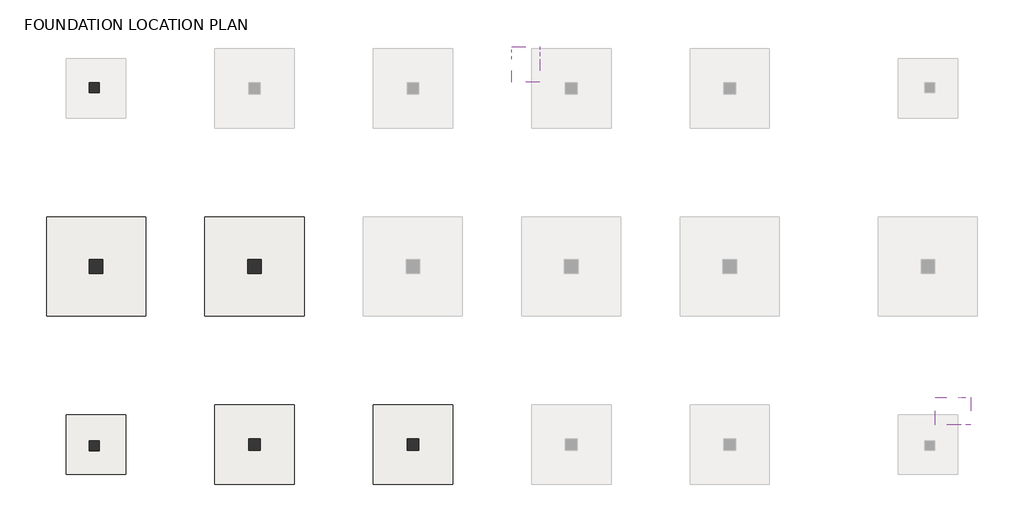
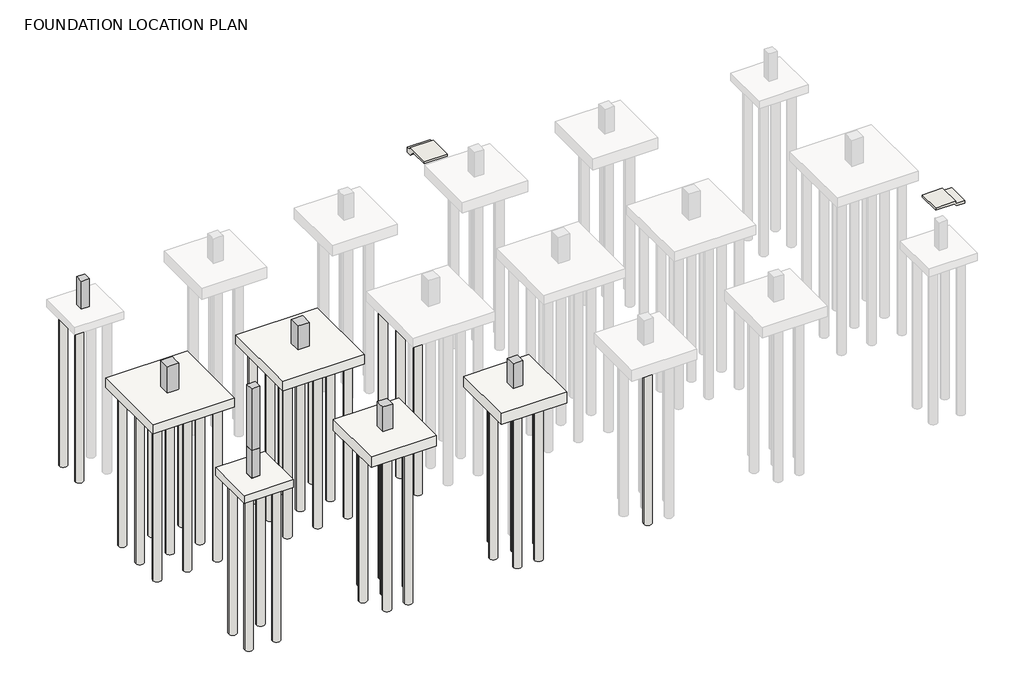
# One storey, part 1 of 3: 46 slabs, 7 columns, 2 walls.
"""IFC4 building model written with IfcOpenShell, lengths in millimetres."""

import ifcopenshell
import ifcopenshell.guid

model = None  # the IFC model being written
_history = None  # IfcOwnerHistory: only IFC2X3 demands one
_inside = {}  # id of a spatial element -> (the spatial element, [elements in it])
_under = {}  # id of a project, library or spatial element -> (it, [spatial elements below it])
_declared = {}  # id of a project -> (the project, [libraries it declares])
_typed = {}  # id of a type object -> (the type object, [elements of that type])
_made_of = {}  # id of a material, layer set ... -> (it, [elements and type objects made of it])


def new_model(schema):
    """Start an empty IFC model of exactly this schema.

    Asked for "IFC4X3", IfcOpenShell would pick the latest addendum, in which some entities
    have other attributes; the version numbers below select the first issue.
    IFC2X3 requires an IfcOwnerHistory on every rooted entity: one is made here for all.
    """
    global model, _history
    if schema == "IFC4X3":
        model = ifcopenshell.file(schema_version=(4, 3, 0, 0))
    else:
        model = ifcopenshell.file(schema=schema)
    _inside.clear()
    _under.clear()
    _declared.clear()
    _typed.clear()
    _made_of.clear()
    _history = None
    if model.schema == "IFC2X3":
        org = make("IfcOrganization", Name="unknown")
        user = make(
            "IfcPersonAndOrganization",
            ThePerson=make("IfcPerson", FamilyName="unknown"),
            TheOrganization=org,
        )
        app = make(
            "IfcApplication",
            ApplicationDeveloper=org,
            Version="unknown",
            ApplicationFullName="unknown",
            ApplicationIdentifier="unknown",
        )
        _history = make(
            "IfcOwnerHistory",
            OwningUser=user,
            OwningApplication=app,
            ChangeAction="ADDED",
            CreationDate=0,
        )
    return model


def make(cls, **values):
    """One entity of the class cls with the attributes given. An attribute that is None is left unset."""
    return model.create_entity(
        cls, **{name: value for name, value in values.items() if value is not None}
    )


def rooted(cls, **values):
    """An entity with a GlobalId (a new one), such as an element, a storey or a relation."""
    return make(cls, GlobalId=ifcopenshell.guid.new(), OwnerHistory=_history, **values)


def si_unit(unit_type, name, prefix=None):
    """IfcSIUnit, for example si_unit("LENGTHUNIT", "METRE", prefix="MILLI")."""
    return make("IfcSIUnit", UnitType=unit_type, Prefix=prefix, Name=name)


def assignment(units):
    """IfcUnitAssignment: the units of a project."""
    return None if units is None else make("IfcUnitAssignment", Units=units)


def point(xyz):
    """IfcCartesianPoint."""
    return None if xyz is None else make("IfcCartesianPoint", Coordinates=xyz)


def direction(xyz):
    """IfcDirection."""
    return None if xyz is None else make("IfcDirection", DirectionRatios=xyz)


def frame(location, z_axis=None, x_axis=None):
    """IfcAxis2Placement3D, a coordinate frame: its origin and axes. An axis left out is left unset."""
    return make(
        "IfcAxis2Placement3D",
        Location=point(location),
        Axis=direction(z_axis),
        RefDirection=direction(x_axis),
    )


def frame_2d(location, x_axis=None):
    """IfcAxis2Placement2D, a coordinate frame in the plane: its origin and x axis."""
    return make(
        "IfcAxis2Placement2D", Location=point(location), RefDirection=direction(x_axis)
    )


def origin():
    """The frame at (0, 0, 0) with its axes left unset."""
    return frame((0.0, 0.0, 0.0))


def place(relative_to, where):
    """IfcLocalPlacement: puts the frame where relative to a parent placement (None: the world)."""
    return make(
        "IfcLocalPlacement", PlacementRelTo=relative_to, RelativePlacement=where
    )


def context(
    kind, dimensions, precision=None, world=None, true_north=None, identifier=None
):
    """IfcGeometricRepresentationContext, for example the 3D "Model" context."""
    return make(
        "IfcGeometricRepresentationContext",
        ContextIdentifier=identifier,
        ContextType=kind,
        CoordinateSpaceDimension=dimensions,
        Precision=precision,
        WorldCoordinateSystem=world,
        TrueNorth=true_north,
    )


def project(units=None, contexts=None):
    """IfcProject with its units and contexts."""
    return rooted(
        "IfcProject",
        Name="project",
        RepresentationContexts=contexts,
        UnitsInContext=assignment(units),
    )


def spatial(cls, under=None, at=None, **own):
    """A site, building, storey or space (cls), placed at a placement, below another one or the project."""
    s = rooted(cls, ObjectPlacement=at, **own)
    if under is not None:
        _under.setdefault(under.id(), (under, []))[1].append(s)
    return s


def polyline(points):
    """IfcPolyline through the points."""
    return make("IfcPolyline", Points=[point(p) for p in points])


def circle_curve(where, radius):
    """IfcCircle in the frame where."""
    return make("IfcCircle", Position=where, Radius=radius)


def trimmed(basis, trim1, trim2, sense, master):
    """IfcTrimmedCurve: the piece of a basis curve between two trims."""
    return make(
        "IfcTrimmedCurve",
        BasisCurve=basis,
        Trim1=trim1,
        Trim2=trim2,
        SenseAgreement=sense,
        MasterRepresentation=master,
    )


def segment(curve, same_sense, transition):
    """IfcCompositeCurveSegment."""
    return make(
        "IfcCompositeCurveSegment",
        Transition=transition,
        SameSense=same_sense,
        ParentCurve=curve,
    )


def composite_curve(segments, self_intersect=None):
    """IfcCompositeCurve: segments joined end to end."""
    return make("IfcCompositeCurve", Segments=segments, SelfIntersect=self_intersect)


def outline(outer, holes=None, kind="AREA"):
    """IfcArbitraryClosedProfileDef: a profile drawn as a closed curve; with holes, ...WithVoids."""
    if holes is None:
        return make("IfcArbitraryClosedProfileDef", ProfileType=kind, OuterCurve=outer)
    return make(
        "IfcArbitraryProfileDefWithVoids",
        ProfileType=kind,
        OuterCurve=outer,
        InnerCurves=holes,
    )


def extrude(swept, where, along, depth):
    """IfcExtrudedAreaSolid: the profile swept, set in the frame where, extruded along a direction by depth."""
    return make(
        "IfcExtrudedAreaSolid",
        SweptArea=swept,
        Position=where,
        ExtrudedDirection=direction(along),
        Depth=depth,
    )


def faces_of(points, faces, orient=None, outer=None):
    """IfcFace entities. A face is a list of loops; a loop is a list of indices into points, from 0.

    orient and outer hold one flag for each loop. By default every Orientation is true, the
    first loop of a face is its IfcFaceOuterBound and the others are IfcFaceBound.
    """
    made = []
    for i, loops in enumerate(faces):
        bounds = []
        for j, loop in enumerate(loops):
            is_outer = j == 0 if outer is None else outer[i][j]
            bounds.append(
                make(
                    "IfcFaceOuterBound" if is_outer else "IfcFaceBound",
                    Bound=make("IfcPolyLoop", Polygon=[points[k] for k in loop]),
                    Orientation=True if orient is None else orient[i][j],
                )
            )
        made.append(make("IfcFace", Bounds=bounds))
    return made


def faceted_brep(points, faces, orient=None, outer=None, voids=None):
    """IfcFacetedBrep: a solid bounded by flat faces; with voids (closed shells), ...WithVoids."""
    shared = [point(p) for p in points]
    hull = make("IfcClosedShell", CfsFaces=faces_of(shared, faces, orient, outer))
    if voids is None:
        return make("IfcFacetedBrep", Outer=hull)
    return make(
        "IfcFacetedBrepWithVoids",
        Outer=hull,
        Voids=[
            make(cls, CfsFaces=faces_of(shared, fs, o, b)) for cls, fs, o, b in voids
        ],
    )


def shape(context_of_items, identifier, shape_type, items):
    """IfcShapeRepresentation: the items that make up one representation, for example the "Body"."""
    return make(
        "IfcShapeRepresentation",
        ContextOfItems=context_of_items,
        RepresentationIdentifier=identifier,
        RepresentationType=shape_type,
        Items=items,
    )


def source(mapping_origin, context_of_items, identifier, shape_type, items):
    """IfcRepresentationMap: a shape defined once, which mapped items show again and again."""
    return make(
        "IfcRepresentationMap",
        MappingOrigin=mapping_origin,
        MappedRepresentation=shape(context_of_items, identifier, shape_type, items),
    )


def transform(
    local_origin,
    x_axis=None,
    y_axis=None,
    z_axis=None,
    scale=None,
    scale2=None,
    scale3=None,
    uniform=True,
):
    """IfcCartesianTransformationOperator3D, or its non-uniform kind. x_axis, y_axis, z_axis: its Axis1, 2, 3."""
    if uniform:
        return make(
            "IfcCartesianTransformationOperator3D",
            Axis1=direction(x_axis),
            Axis2=direction(y_axis),
            LocalOrigin=point(local_origin),
            Scale=scale,
            Axis3=direction(z_axis),
        )
    return make(
        "IfcCartesianTransformationOperator3DnonUniform",
        Axis1=direction(x_axis),
        Axis2=direction(y_axis),
        LocalOrigin=point(local_origin),
        Scale=scale,
        Axis3=direction(z_axis),
        Scale2=scale2,
        Scale3=scale3,
    )


def mapped(mapping_source, mapping_target):
    """IfcMappedItem: shows the shape of a source again, moved by a transform."""
    return make(
        "IfcMappedItem", MappingSource=mapping_source, MappingTarget=mapping_target
    )


def made_of(thing, what):
    """Note that an element or type object is made of a material, layer set ...; save() writes the relation."""
    if what is not None:
        _made_of.setdefault(what.id(), (what, []))[1].append(thing)
    return thing


def element(
    cls,
    number,
    at=None,
    inside=None,
    cuts=None,
    type_object=None,
    material=None,
    context=None,
    identifier="Body",
    shape_type=None,
    held_by="IfcProductDefinitionShape",
    body=None,
    shapes=None,
    **own,
):
    """One element of the class cls, such as IfcWall. Its Tag is "e" and its number.

    at: its placement. inside: the storey or other place that contains it. cuts: it is an
    opening in that element (IfcRelVoidsElement). A single representation is given by context,
    identifier, shape_type and body (its items); several are given by shapes. held_by: the class
    of the entity that holds the representations. save() writes the other relations.
    """
    e = rooted(cls, Tag="e%d" % number, ObjectPlacement=at, **own)
    if body is not None:
        shapes = [shape(context, identifier, shape_type, body)]
    if shapes is not None:
        e.Representation = make(held_by, Representations=shapes)
    if inside is not None:
        _inside.setdefault(inside.id(), (inside, []))[1].append(e)
    if cuts is not None:
        rooted(
            "IfcRelVoidsElement", RelatingBuildingElement=cuts, RelatedOpeningElement=e
        )
    if type_object is not None:
        _typed.setdefault(type_object.id(), (type_object, []))[1].append(e)
    return made_of(e, material)


def aggregate(whole, parts):
    """IfcRelAggregates: a whole, such as a stair, and the parts it consists of."""
    return rooted("IfcRelAggregates", RelatingObject=whole, RelatedObjects=parts)


def save(model, path):
    """Write the relations noted so far, then the file.

    IfcRelAggregates (storeys below a building ...), IfcRelContainedInSpatialStructure (elements
    in a storey), IfcRelDefinesByType, IfcRelAssociatesMaterial and IfcRelDeclares: one each for
    every whole, place, type object, material and project.
    """
    for whole, parts in _under.values():
        aggregate(whole, parts)
    for where, things in _inside.values():
        rooted(
            "IfcRelContainedInSpatialStructure",
            RelatedElements=things,
            RelatingStructure=where,
        )
    for kind, things in _typed.values():
        rooted("IfcRelDefinesByType", RelatedObjects=things, RelatingType=kind)
    for what, things in _made_of.values():
        rooted("IfcRelAssociatesMaterial", RelatedObjects=things, RelatingMaterial=what)
    for by, libraries in _declared.values():
        rooted("IfcRelDeclares", RelatingContext=by, RelatedDefinitions=libraries)
    model.write(path)


def wall_a06d278e(model_context):
    return source(origin(), model_context, "Body", "SweptSolid", [
        extrude(outline(polyline([(599.905241, 43602.1335861), (599.905241, 42370.0), (449.905241, 42370.0), (449.905241, 43520.0), (299.905241, 43670.0), (299.905241, 44170.4893475), (449.905241, 44170.4893475), (449.905241, 43602.1335861), (599.905241, 43602.1335861)])), frame((0.0, 21999.5208589, 0.0), z_axis=(0.0, 1.0, 0.0), x_axis=(0.0, 0.0, 1.0)), (0.0, 0.0, 1.0), 1400.0),
    ])


def wall_c40cd3bd(model_context):
    return source(origin(), model_context, "Body", "SweptSolid", [
        extrude(outline(polyline([(40819.5208589, 599.905241), (40819.5208589, 449.905241), (41119.5208589, 449.905241), (41119.5208589, 109.2314637), (40810.1946362, 109.2314637), (40469.5208589, 449.905241), (39319.5208589, 449.905241), (39319.5208589, 599.905241), (40819.5208589, 599.905241)])), frame((21000.0, 0.0, 0.0), z_axis=(1.0, 0.0, 0.0), x_axis=(0.0, 1.0, 0.0)), (0.0, 0.0, 1.0), 1400.0),
    ])


model = new_model("IFC4")

# Units and contexts
model_context = context("Model", 3, world=origin())
ifc_project = project(units=[si_unit("LENGTHUNIT", "METRE", prefix="MILLI")], contexts=[model_context])

# Site, building, storey
site = spatial("IfcSite", under=ifc_project)
building = spatial("IfcBuilding", under=site)
storey = spatial("IfcBuildingStorey", under=building, Name="FOUNDATION LOCATION PLAN", Elevation=-1699.994759)

# Columns
placement = place(None, origin())
element("IfcColumn", 1, ObjectType="Concrete-Rectangular-Column_R1 : CLS113_RC COLUMN_AG_C1", at=placement, inside=storey, context=model_context, shape_type="Brep", body=[
    faceted_brep([(-350.0, 21199.5208589, -1699.994759), (150.0, 21199.5208589, -1699.994759), (150.0, 20699.5208589, -1699.994759), (-350.0, 20699.5208589, -1699.994759), (150.0, 21199.5208589, -1199.994759), (-350.0, 21199.5208589, -1199.994759), (-350.0, 20699.5208589, -1199.994759), (150.0, 20699.5208589, -1199.994759)], [[[0, 1, 2, 3]], [[4, 5, 6, 7]], [[1, 0, 5, 4]], [[2, 1, 4, 7]], [[3, 2, 7, 6]], [[0, 3, 6, 5]]]),
    faceted_brep([(-350.0, 21199.5208589, 4600.005241), (150.0, 21199.5208589, 4600.005241), (150.0, 21199.5208589, 600.005241), (-99.0, 21199.5208589, 600.005241), (-350.0, 21199.5208589, 600.005241), (-350.0, 21199.5208589, 3950.005241), (-350.0, 21199.5208589, 4550.005241), (150.0, 20699.5208589, 4600.005241), (150.0, 20699.5208589, 4550.005241), (150.0, 20699.5208589, 3950.005241), (150.0, 20699.5208589, 600.005241), (150.0, 20950.5208589, 600.005241), (-350.0, 20699.5208589, 4600.005241), (-350.0, 20699.5208589, 4550.005241), (-350.0, 20699.5208589, 3950.005241), (-350.0, 20699.5208589, 600.005241)], [[[0, 1, 2, 3, 4, 5, 6]], [[1, 7, 8, 9, 10, 11, 2]], [[7, 12, 13, 14, 15, 10, 9, 8]], [[12, 0, 6, 5, 4, 15, 14, 13]], [[1, 0, 12, 7]], [[4, 3, 2, 11, 10, 15]]]),
])
element("IfcColumn", 2, ObjectType="Concrete-Rectangular-Column_R1 : CLS111_RC COLUMN_UG_C1", at=placement, inside=storey, context=model_context, shape_type="Brep", body=[
    faceted_brep([(-350.0, 21199.5208589, -1199.994759), (150.0, 21199.5208589, -1199.994759), (150.0, 20699.5208589, -1199.994759), (-350.0, 20699.5208589, -1199.994759), (-350.0, 21199.5208589, 450.005241), (-350.0, 21199.5208589, 600.005241), (150.0, 21199.5208589, 600.005241), (150.0, 21199.5208589, 450.005241), (150.0, 20699.5208589, 600.005241), (150.0, 20699.5208589, 450.005241), (-350.0, 20699.5208589, 600.005241)], [[[0, 1, 2, 3]], [[1, 0, 4, 5, 6, 7]], [[2, 1, 7, 6, 8, 9]], [[3, 2, 9, 8, 10]], [[0, 3, 10, 5, 4]], [[6, 5, 10, 8]]]),
])
element("IfcColumn", 3, ObjectType="Concrete-Rectangular-Column_R1 : CLS111_RC COLUMN_UG_C1", at=placement, inside=storey, context=model_context, shape_type="Brep", body=[
    faceted_brep([(-350.0, 39299.5208589, -1199.994759), (150.0, 39299.5208589, -1199.994759), (150.0, 38799.5208589, -1199.994759), (-350.0, 38799.5208589, -1199.994759), (-350.0, 39299.5208589, 600.005241), (150.0, 39299.5208589, 600.005241), (150.0, 38999.7368538, 600.005241), (150.0, 38799.7368538, 600.005241), (150.0, 38799.5208589, 600.005241), (150.0, 38799.5208589, 450.005241), (0.0, 38799.5208589, 600.005241), (-350.0, 38799.5208589, 600.005241), (-350.0, 38799.7368538, 600.005241)], [[[0, 1, 2, 3]], [[1, 0, 4, 5]], [[2, 1, 5, 6, 7, 8, 9]], [[3, 2, 9, 8, 10, 11]], [[0, 3, 11, 12, 4]], [[5, 4, 12, 11, 10, 8, 7, 6]]]),
])
element("IfcColumn", 4, ObjectType="Concrete-Rectangular-Column_R1 : CLS111_RC COLUMN_UG_C3", at=placement, inside=storey, context=model_context, shape_type="Brep", body=[
    faceted_brep([(-350.0, 30349.5208589, -1099.994759), (350.0, 30349.5208589, -1099.994759), (350.0, 29649.5208589, -1099.994759), (-350.0, 29649.5208589, -1099.994759), (-350.0, 30349.5208589, 600.005241), (0.0, 30349.5208589, 600.005241), (350.0, 30349.5208589, 600.005241), (350.0, 30349.5208589, 450.005241), (350.0, 29999.5208589, 600.005241), (350.0, 29649.5208589, 600.005241), (-99.0, 29649.5208589, 600.005241), (-350.0, 29649.5208589, 600.005241)], [[[0, 1, 2, 3]], [[1, 0, 4, 5, 6, 7]], [[2, 1, 7, 6, 8, 9]], [[3, 2, 9, 10, 11]], [[0, 3, 11, 4]], [[11, 10, 9, 8, 6, 5, 4]]]),
])
element("IfcColumn", 5, ObjectType="Concrete-Rectangular-Column_R1 : CLS111_RC COLUMN_UG_C3", at=placement, inside=storey, context=model_context, shape_type="SweptSolid", body=[
    extrude(outline(polyline([(7650.0, 30349.5208589), (8350.0, 30349.5208589), (8350.0, 29649.5208589), (7650.0, 29649.5208589), (7650.0, 30349.5208589)])), frame((0.0, 0.0, -1099.994759), z_axis=(0.0, 0.0, 1.0), x_axis=(1.0, 0.0, 0.0)), (0.0, 0.0, 1.0), 1550.0),
])
element("IfcColumn", 6, ObjectType="Concrete-Rectangular-Column_R1 : CLS111_RC COLUMN_UG_C2", at=placement, inside=storey, context=model_context, shape_type="Brep", body=[
    faceted_brep([(7700.0, 21299.5208589, -999.994759), (8300.0, 21299.5208589, -999.994759), (8300.0, 20699.5208589, -999.994759), (7700.0, 20699.5208589, -999.994759), (7700.0, 21299.5208589, 450.005241), (7700.0, 21299.5208589, 600.005241), (8300.0, 21299.5208589, 600.005241), (8300.0, 21299.5208589, 450.005241), (8300.0, 20999.5208589, 600.005241), (8300.0, 20699.5208589, 600.005241), (7700.0, 20699.5208589, 600.005241), (7700.0, 20999.5208589, 600.005241)], [[[0, 1, 2, 3]], [[1, 0, 4, 5, 6, 7]], [[2, 1, 7, 6, 8, 9]], [[3, 2, 9, 10]], [[0, 3, 10, 11, 5, 4]], [[6, 5, 11, 10, 9, 8]]]),
])
element("IfcColumn", 7, ObjectType="Concrete-Rectangular-Column_R1 : CLS111_RC COLUMN_UG_C2", at=placement, inside=storey, context=model_context, shape_type="Brep", body=[
    faceted_brep([(15700.0, 21299.5208589, -999.994759), (16300.0, 21299.5208589, -999.994759), (16300.0, 20699.5208589, -999.994759), (15700.0, 20699.5208589, -999.994759), (15700.0, 21299.5208589, 450.005241), (15700.0, 21299.5208589, 600.005241), (16300.0, 21299.5208589, 600.005241), (16300.0, 21299.5208589, 450.005241), (16300.0, 20999.5208589, 600.005241), (16300.0, 20699.5208589, 600.005241), (15700.0, 20699.5208589, 600.005241), (15700.0, 20999.5208589, 600.005241)], [[[0, 1, 2, 3]], [[1, 0, 4, 5, 6, 7]], [[2, 1, 7, 6, 8, 9]], [[3, 2, 9, 10]], [[0, 3, 10, 11, 5, 4]], [[6, 5, 11, 10, 9, 8]]]),
])

# Slabs
element("IfcSlab", 8, ObjectType="Footing-Rectangular_R1 : FTS301_Footing-Rectangular_3000x3000x500_F1", at=placement, inside=storey, context=model_context, shape_type="SweptSolid", body=[
    extrude(outline(polyline([(1500.0, 22499.5208589), (1500.0, 19499.5208589), (-1500.0, 19499.5208589), (-1500.0, 22499.5208589), (1500.0, 22499.5208589)])), frame((0.0, 0.0, -1699.994759), z_axis=(0.0, 0.0, 1.0), x_axis=(1.0, 0.0, 0.0)), (0.0, 0.0, 1.0), 500.0),
])
element("IfcSlab", 9, ObjectType="Footing-Rectangular_R1 : FTS301_Footing-Rectangular_4000x4000x700_F2", at=placement, inside=storey, context=model_context, shape_type="SweptSolid", body=[
    extrude(outline(polyline([(10000.0, 22999.5208589), (10000.0, 18999.5208589), (6000.0, 18999.5208589), (6000.0, 22999.5208589), (10000.0, 22999.5208589)])), frame((0.0, 0.0, -1699.994759), z_axis=(0.0, 0.0, 1.0), x_axis=(1.0, 0.0, 0.0)), (0.0, 0.0, 1.0), 700.0),
])
element("IfcSlab", 10, ObjectType="Footing-Rectangular_R1 : FTS301_Footing-Rectangular_4000x4000x700_F2", at=placement, inside=storey, context=model_context, shape_type="SweptSolid", body=[
    extrude(outline(polyline([(18000.0, 22999.5208589), (18000.0, 18999.5208589), (14000.0, 18999.5208589), (14000.0, 22999.5208589), (18000.0, 22999.5208589)])), frame((0.0, 0.0, -1699.994759), z_axis=(0.0, 0.0, 1.0), x_axis=(1.0, 0.0, 0.0)), (0.0, 0.0, 1.0), 700.0),
])
element("IfcSlab", 11, ObjectType="Footing-Rectangular_R1 : FTS301_Footing-Rectangular_5000x5000x600_F3", at=placement, inside=storey, context=model_context, shape_type="SweptSolid", body=[
    extrude(outline(polyline([(2500.0, 32499.5208589), (2500.0, 27499.5208589), (-2500.0, 27499.5208589), (-2500.0, 32499.5208589), (2500.0, 32499.5208589)])), frame((0.0, 0.0, -1699.994759), z_axis=(0.0, 0.0, 1.0), x_axis=(1.0, 0.0, 0.0)), (0.0, 0.0, 1.0), 600.0),
])
element("IfcSlab", 12, ObjectType="Footing-Rectangular_R1 : FTS301_Footing-Rectangular_5000x5000x600_F3", at=placement, inside=storey, context=model_context, shape_type="SweptSolid", body=[
    extrude(outline(polyline([(10500.0, 32499.5208589), (10500.0, 27499.5208589), (5500.0, 27499.5208589), (5500.0, 32499.5208589), (10500.0, 32499.5208589)])), frame((0.0, 0.0, -1699.994759), z_axis=(0.0, 0.0, 1.0), x_axis=(1.0, 0.0, 0.0)), (0.0, 0.0, 1.0), 600.0),
])
element("IfcSlab", 13, ObjectType="HEC_PILE : FTPS102_D500", at=placement, inside=storey, context=model_context, shape_type="SweptSolid", body=[
    extrude(outline(composite_curve([segment(trimmed(circle_curve(frame_2d((7350.0, 19649.5208589)), 250.0), [point((7600.0, 19649.5208589))], [point((7100.0, 19649.5208589))], False, "CARTESIAN"), True, "CONTINUOUS"), segment(trimmed(circle_curve(frame_2d((7350.0, 19649.5208589)), 250.0), [point((7100.0, 19649.5208589))], [point((7600.0, 19649.5208589))], False, "CARTESIAN"), True, "CONTINUOUS")], self_intersect=False)), frame((0.0, 0.0, -11749.994759), z_axis=(0.0, 0.0, 1.0), x_axis=(1.0, 0.0, 0.0)), (0.0, 0.0, 1.0), 10150.0),
])
element("IfcSlab", 14, ObjectType="HEC_PILE : FTPS102_D500", at=placement, inside=storey, context=model_context, shape_type="SweptSolid", body=[
    extrude(outline(composite_curve([segment(trimmed(circle_curve(frame_2d((8650.0, 19649.5208589)), 250.0), [point((8400.0, 19649.5208589))], [point((8900.0, 19649.5208589))], False, "CARTESIAN"), True, "CONTINUOUS"), segment(trimmed(circle_curve(frame_2d((8650.0, 19649.5208589)), 250.0), [point((8900.0, 19649.5208589))], [point((8400.0, 19649.5208589))], False, "CARTESIAN"), True, "CONTINUOUS")], self_intersect=False)), frame((0.0, 0.0, -11749.994759), z_axis=(0.0, 0.0, 1.0), x_axis=(1.0, 0.0, 0.0)), (0.0, 0.0, 1.0), 10150.0),
])
element("IfcSlab", 15, ObjectType="HEC_PILE : FTPS102_D500", at=placement, inside=storey, context=model_context, shape_type="SweptSolid", body=[
    extrude(outline(composite_curve([segment(trimmed(circle_curve(frame_2d((6650.0, 20999.5208589)), 250.0), [point((6900.0, 20999.5208589))], [point((6400.0, 20999.5208589))], False, "CARTESIAN"), True, "CONTINUOUS"), segment(trimmed(circle_curve(frame_2d((6650.0, 20999.5208589)), 250.0), [point((6400.0, 20999.5208589))], [point((6900.0, 20999.5208589))], False, "CARTESIAN"), True, "CONTINUOUS")], self_intersect=False)), frame((0.0, 0.0, -11749.994759), z_axis=(0.0, 0.0, 1.0), x_axis=(1.0, 0.0, 0.0)), (0.0, 0.0, 1.0), 10150.0),
])
element("IfcSlab", 16, ObjectType="HEC_PILE : FTPS102_D500", at=placement, inside=storey, context=model_context, shape_type="SweptSolid", body=[
    extrude(outline(composite_curve([segment(trimmed(circle_curve(frame_2d((8000.0, 20999.5208589)), 250.0), [point((8250.0, 20999.5208589))], [point((7750.0, 20999.5208589))], False, "CARTESIAN"), True, "CONTINUOUS"), segment(trimmed(circle_curve(frame_2d((8000.0, 20999.5208589)), 250.0), [point((7750.0, 20999.5208589))], [point((8250.0, 20999.5208589))], False, "CARTESIAN"), True, "CONTINUOUS")], self_intersect=False)), frame((0.0, 0.0, -11749.994759), z_axis=(0.0, 0.0, 1.0), x_axis=(1.0, 0.0, 0.0)), (0.0, 0.0, 1.0), 10150.0),
])
element("IfcSlab", 17, ObjectType="HEC_PILE : FTPS102_D500", at=placement, inside=storey, context=model_context, shape_type="SweptSolid", body=[
    extrude(outline(composite_curve([segment(trimmed(circle_curve(frame_2d((9350.0, 20999.5208589)), 250.0), [point((9100.0, 20999.5208589))], [point((9600.0, 20999.5208589))], False, "CARTESIAN"), True, "CONTINUOUS"), segment(trimmed(circle_curve(frame_2d((9350.0, 20999.5208589)), 250.0), [point((9600.0, 20999.5208589))], [point((9100.0, 20999.5208589))], False, "CARTESIAN"), True, "CONTINUOUS")], self_intersect=False)), frame((0.0, 0.0, -11749.994759), z_axis=(0.0, 0.0, 1.0), x_axis=(1.0, 0.0, 0.0)), (0.0, 0.0, 1.0), 10150.0),
])
element("IfcSlab", 18, ObjectType="HEC_PILE : FTPS102_D500", at=placement, inside=storey, context=model_context, shape_type="SweptSolid", body=[
    extrude(outline(composite_curve([segment(trimmed(circle_curve(frame_2d((7350.0, 22349.5208589)), 250.0), [point((7600.0, 22349.5208589))], [point((7100.0, 22349.5208589))], False, "CARTESIAN"), True, "CONTINUOUS"), segment(trimmed(circle_curve(frame_2d((7350.0, 22349.5208589)), 250.0), [point((7100.0, 22349.5208589))], [point((7600.0, 22349.5208589))], False, "CARTESIAN"), True, "CONTINUOUS")], self_intersect=False)), frame((0.0, 0.0, -11749.994759), z_axis=(0.0, 0.0, 1.0), x_axis=(1.0, 0.0, 0.0)), (0.0, 0.0, 1.0), 10150.0),
])
element("IfcSlab", 19, ObjectType="HEC_PILE : FTPS102_D500", at=placement, inside=storey, context=model_context, shape_type="SweptSolid", body=[
    extrude(outline(composite_curve([segment(trimmed(circle_curve(frame_2d((8650.0, 22349.5208589)), 250.0), [point((8400.0, 22349.5208589))], [point((8900.0, 22349.5208589))], False, "CARTESIAN"), True, "CONTINUOUS"), segment(trimmed(circle_curve(frame_2d((8650.0, 22349.5208589)), 250.0), [point((8900.0, 22349.5208589))], [point((8400.0, 22349.5208589))], False, "CARTESIAN"), True, "CONTINUOUS")], self_intersect=False)), frame((0.0, 0.0, -11749.994759), z_axis=(0.0, 0.0, 1.0), x_axis=(1.0, 0.0, 0.0)), (0.0, 0.0, 1.0), 10150.0),
])
element("IfcSlab", 20, ObjectType="HEC_PILE : FTPS102_D500", at=placement, inside=storey, context=model_context, shape_type="SweptSolid", body=[
    extrude(outline(composite_curve([segment(trimmed(circle_curve(frame_2d((-850.0, 39849.5208589)), 250.0), [point((-600.0, 39849.5208589))], [point((-1100.0, 39849.5208589))], False, "CARTESIAN"), True, "CONTINUOUS"), segment(trimmed(circle_curve(frame_2d((-850.0, 39849.5208589)), 250.0), [point((-1100.0, 39849.5208589))], [point((-600.0, 39849.5208589))], False, "CARTESIAN"), True, "CONTINUOUS")], self_intersect=False)), frame((0.0, 0.0, -11749.994759), z_axis=(0.0, 0.0, 1.0), x_axis=(1.0, 0.0, 0.0)), (0.0, 0.0, 1.0), 10150.0),
])
element("IfcSlab", 21, ObjectType="HEC_PILE : FTPS102_D500", at=placement, inside=storey, context=model_context, shape_type="SweptSolid", body=[
    extrude(outline(composite_curve([segment(trimmed(circle_curve(frame_2d((-850.0, 21849.5208589)), 250.0), [point((-600.0, 21849.5208589))], [point((-1100.0, 21849.5208589))], False, "CARTESIAN"), True, "CONTINUOUS"), segment(trimmed(circle_curve(frame_2d((-850.0, 21849.5208589)), 250.0), [point((-1100.0, 21849.5208589))], [point((-600.0, 21849.5208589))], False, "CARTESIAN"), True, "CONTINUOUS")], self_intersect=False)), frame((0.0, 0.0, -11749.994759), z_axis=(0.0, 0.0, 1.0), x_axis=(1.0, 0.0, 0.0)), (0.0, 0.0, 1.0), 10150.0),
])
element("IfcSlab", 22, ObjectType="HEC_PILE : FTPS102_D500", at=placement, inside=storey, context=model_context, shape_type="SweptSolid", body=[
    extrude(outline(composite_curve([segment(trimmed(circle_curve(frame_2d((850.0, 21849.5208589)), 250.0), [point((600.0, 21849.5208589))], [point((1100.0, 21849.5208589))], False, "CARTESIAN"), True, "CONTINUOUS"), segment(trimmed(circle_curve(frame_2d((850.0, 21849.5208589)), 250.0), [point((1100.0, 21849.5208589))], [point((600.0, 21849.5208589))], False, "CARTESIAN"), True, "CONTINUOUS")], self_intersect=False)), frame((0.0, 0.0, -11749.994759), z_axis=(0.0, 0.0, 1.0), x_axis=(1.0, 0.0, 0.0)), (0.0, 0.0, 1.0), 10150.0),
])
element("IfcSlab", 23, ObjectType="HEC_PILE : FTPS102_D500", at=placement, inside=storey, context=model_context, shape_type="SweptSolid", body=[
    extrude(outline(composite_curve([segment(trimmed(circle_curve(frame_2d((-850.0, 20149.5208589)), 250.0), [point((-600.0, 20149.5208589))], [point((-1100.0, 20149.5208589))], False, "CARTESIAN"), True, "CONTINUOUS"), segment(trimmed(circle_curve(frame_2d((-850.0, 20149.5208589)), 250.0), [point((-1100.0, 20149.5208589))], [point((-600.0, 20149.5208589))], False, "CARTESIAN"), True, "CONTINUOUS")], self_intersect=False)), frame((0.0, 0.0, -11749.994759), z_axis=(0.0, 0.0, 1.0), x_axis=(1.0, 0.0, 0.0)), (0.0, 0.0, 1.0), 10150.0),
])
element("IfcSlab", 24, ObjectType="HEC_PILE : FTPS102_D500", at=placement, inside=storey, context=model_context, shape_type="SweptSolid", body=[
    extrude(outline(composite_curve([segment(trimmed(circle_curve(frame_2d((850.0, 20149.5208589)), 250.0), [point((600.0, 20149.5208589))], [point((1100.0, 20149.5208589))], False, "CARTESIAN"), True, "CONTINUOUS"), segment(trimmed(circle_curve(frame_2d((850.0, 20149.5208589)), 250.0), [point((1100.0, 20149.5208589))], [point((600.0, 20149.5208589))], False, "CARTESIAN"), True, "CONTINUOUS")], self_intersect=False)), frame((0.0, 0.0, -11749.994759), z_axis=(0.0, 0.0, 1.0), x_axis=(1.0, 0.0, 0.0)), (0.0, 0.0, 1.0), 10150.0),
])
element("IfcSlab", 25, ObjectType="HEC_PILE : FTPS102_D500", at=placement, inside=storey, context=model_context, shape_type="SweptSolid", body=[
    extrude(outline(composite_curve([segment(trimmed(circle_curve(frame_2d((15350.0, 19649.5208589)), 250.0), [point((15600.0, 19649.5208589))], [point((15100.0, 19649.5208589))], False, "CARTESIAN"), True, "CONTINUOUS"), segment(trimmed(circle_curve(frame_2d((15350.0, 19649.5208589)), 250.0), [point((15100.0, 19649.5208589))], [point((15600.0, 19649.5208589))], False, "CARTESIAN"), True, "CONTINUOUS")], self_intersect=False)), frame((0.0, 0.0, -11749.994759), z_axis=(0.0, 0.0, 1.0), x_axis=(1.0, 0.0, 0.0)), (0.0, 0.0, 1.0), 10150.0),
])
element("IfcSlab", 26, ObjectType="HEC_PILE : FTPS102_D500", at=placement, inside=storey, context=model_context, shape_type="SweptSolid", body=[
    extrude(outline(composite_curve([segment(trimmed(circle_curve(frame_2d((16650.0, 19649.5208589)), 250.0), [point((16400.0, 19649.5208589))], [point((16900.0, 19649.5208589))], False, "CARTESIAN"), True, "CONTINUOUS"), segment(trimmed(circle_curve(frame_2d((16650.0, 19649.5208589)), 250.0), [point((16900.0, 19649.5208589))], [point((16400.0, 19649.5208589))], False, "CARTESIAN"), True, "CONTINUOUS")], self_intersect=False)), frame((0.0, 0.0, -11749.994759), z_axis=(0.0, 0.0, 1.0), x_axis=(1.0, 0.0, 0.0)), (0.0, 0.0, 1.0), 10150.0),
])
element("IfcSlab", 27, ObjectType="HEC_PILE : FTPS102_D500", at=placement, inside=storey, context=model_context, shape_type="SweptSolid", body=[
    extrude(outline(composite_curve([segment(trimmed(circle_curve(frame_2d((14650.0, 20999.5208589)), 250.0), [point((14900.0, 20999.5208589))], [point((14400.0, 20999.5208589))], False, "CARTESIAN"), True, "CONTINUOUS"), segment(trimmed(circle_curve(frame_2d((14650.0, 20999.5208589)), 250.0), [point((14400.0, 20999.5208589))], [point((14900.0, 20999.5208589))], False, "CARTESIAN"), True, "CONTINUOUS")], self_intersect=False)), frame((0.0, 0.0, -11749.994759), z_axis=(0.0, 0.0, 1.0), x_axis=(1.0, 0.0, 0.0)), (0.0, 0.0, 1.0), 10150.0),
])
element("IfcSlab", 28, ObjectType="HEC_PILE : FTPS102_D500", at=placement, inside=storey, context=model_context, shape_type="SweptSolid", body=[
    extrude(outline(composite_curve([segment(trimmed(circle_curve(frame_2d((16000.0, 20999.5208589)), 250.0), [point((16250.0, 20999.5208589))], [point((15750.0, 20999.5208589))], False, "CARTESIAN"), True, "CONTINUOUS"), segment(trimmed(circle_curve(frame_2d((16000.0, 20999.5208589)), 250.0), [point((15750.0, 20999.5208589))], [point((16250.0, 20999.5208589))], False, "CARTESIAN"), True, "CONTINUOUS")], self_intersect=False)), frame((0.0, 0.0, -11749.994759), z_axis=(0.0, 0.0, 1.0), x_axis=(1.0, 0.0, 0.0)), (0.0, 0.0, 1.0), 10150.0),
])
element("IfcSlab", 29, ObjectType="HEC_PILE : FTPS102_D500", at=placement, inside=storey, context=model_context, shape_type="SweptSolid", body=[
    extrude(outline(composite_curve([segment(trimmed(circle_curve(frame_2d((17350.0, 20999.5208589)), 250.0), [point((17100.0, 20999.5208589))], [point((17600.0, 20999.5208589))], False, "CARTESIAN"), True, "CONTINUOUS"), segment(trimmed(circle_curve(frame_2d((17350.0, 20999.5208589)), 250.0), [point((17600.0, 20999.5208589))], [point((17100.0, 20999.5208589))], False, "CARTESIAN"), True, "CONTINUOUS")], self_intersect=False)), frame((0.0, 0.0, -11749.994759), z_axis=(0.0, 0.0, 1.0), x_axis=(1.0, 0.0, 0.0)), (0.0, 0.0, 1.0), 10150.0),
])
element("IfcSlab", 30, ObjectType="HEC_PILE : FTPS102_D500", at=placement, inside=storey, context=model_context, shape_type="SweptSolid", body=[
    extrude(outline(composite_curve([segment(trimmed(circle_curve(frame_2d((15350.0, 22349.5208589)), 250.0), [point((15600.0, 22349.5208589))], [point((15100.0, 22349.5208589))], False, "CARTESIAN"), True, "CONTINUOUS"), segment(trimmed(circle_curve(frame_2d((15350.0, 22349.5208589)), 250.0), [point((15100.0, 22349.5208589))], [point((15600.0, 22349.5208589))], False, "CARTESIAN"), True, "CONTINUOUS")], self_intersect=False)), frame((0.0, 0.0, -11749.994759), z_axis=(0.0, 0.0, 1.0), x_axis=(1.0, 0.0, 0.0)), (0.0, 0.0, 1.0), 10150.0),
])
element("IfcSlab", 31, ObjectType="HEC_PILE : FTPS102_D500", at=placement, inside=storey, context=model_context, shape_type="SweptSolid", body=[
    extrude(outline(composite_curve([segment(trimmed(circle_curve(frame_2d((23350.0, 19649.5208589)), 250.0), [point((23600.0, 19649.5208589))], [point((23100.0, 19649.5208589))], False, "CARTESIAN"), True, "CONTINUOUS"), segment(trimmed(circle_curve(frame_2d((23350.0, 19649.5208589)), 250.0), [point((23100.0, 19649.5208589))], [point((23600.0, 19649.5208589))], False, "CARTESIAN"), True, "CONTINUOUS")], self_intersect=False)), frame((0.0, 0.0, -11749.994759), z_axis=(0.0, 0.0, 1.0), x_axis=(1.0, 0.0, 0.0)), (0.0, 0.0, 1.0), 10150.0),
])
element("IfcSlab", 32, ObjectType="HEC_PILE : FTPS102_D500", at=placement, inside=storey, context=model_context, shape_type="SweptSolid", body=[
    extrude(outline(composite_curve([segment(trimmed(circle_curve(frame_2d((-1850.0, 29999.5208589)), 250.0), [point((-1600.0, 29999.5208589))], [point((-2100.0, 29999.5208589))], False, "CARTESIAN"), True, "CONTINUOUS"), segment(trimmed(circle_curve(frame_2d((-1850.0, 29999.5208589)), 250.0), [point((-2100.0, 29999.5208589))], [point((-1600.0, 29999.5208589))], False, "CARTESIAN"), True, "CONTINUOUS")], self_intersect=False)), frame((0.0, 0.0, -11749.994759), z_axis=(0.0, 0.0, 1.0), x_axis=(1.0, 0.0, 0.0)), (0.0, 0.0, 1.0), 10150.0),
])
element("IfcSlab", 33, ObjectType="HEC_PILE : FTPS102_D500", at=placement, inside=storey, context=model_context, shape_type="SweptSolid", body=[
    extrude(outline(composite_curve([segment(trimmed(circle_curve(frame_2d((1850.0, 29999.5208589)), 250.0), [point((1600.0, 29999.5208589))], [point((2100.0, 29999.5208589))], False, "CARTESIAN"), True, "CONTINUOUS"), segment(trimmed(circle_curve(frame_2d((1850.0, 29999.5208589)), 250.0), [point((2100.0, 29999.5208589))], [point((1600.0, 29999.5208589))], False, "CARTESIAN"), True, "CONTINUOUS")], self_intersect=False)), frame((0.0, 0.0, -11749.994759), z_axis=(0.0, 0.0, 1.0), x_axis=(1.0, 0.0, 0.0)), (0.0, 0.0, 1.0), 10150.0),
])
element("IfcSlab", 34, ObjectType="HEC_PILE : FTPS102_D500", at=placement, inside=storey, context=model_context, shape_type="SweptSolid", body=[
    extrude(outline(composite_curve([segment(trimmed(circle_curve(frame_2d((0.0, 29999.5208589)), 250.0), [point((-250.0, 29999.5208589))], [point((250.0, 29999.5208589))], False, "CARTESIAN"), True, "CONTINUOUS"), segment(trimmed(circle_curve(frame_2d((0.0, 29999.5208589)), 250.0), [point((250.0, 29999.5208589))], [point((-250.0, 29999.5208589))], False, "CARTESIAN"), True, "CONTINUOUS")], self_intersect=False)), frame((0.0, 0.0, -11749.994759), z_axis=(0.0, 0.0, 1.0), x_axis=(1.0, 0.0, 0.0)), (0.0, 0.0, 1.0), 10150.0),
])
element("IfcSlab", 35, ObjectType="HEC_PILE : FTPS102_D500", at=placement, inside=storey, context=model_context, shape_type="SweptSolid", body=[
    extrude(outline(composite_curve([segment(trimmed(circle_curve(frame_2d((-1850.0, 31849.5208589)), 250.0), [point((-1600.0, 31849.5208589))], [point((-2100.0, 31849.5208589))], False, "CARTESIAN"), True, "CONTINUOUS"), segment(trimmed(circle_curve(frame_2d((-1850.0, 31849.5208589)), 250.0), [point((-2100.0, 31849.5208589))], [point((-1600.0, 31849.5208589))], False, "CARTESIAN"), True, "CONTINUOUS")], self_intersect=False)), frame((0.0, 0.0, -11749.994759), z_axis=(0.0, 0.0, 1.0), x_axis=(1.0, 0.0, 0.0)), (0.0, 0.0, 1.0), 10150.0),
])
element("IfcSlab", 36, ObjectType="HEC_PILE : FTPS102_D500", at=placement, inside=storey, context=model_context, shape_type="SweptSolid", body=[
    extrude(outline(composite_curve([segment(trimmed(circle_curve(frame_2d((1850.0, 31849.5208589)), 250.0), [point((1600.0, 31849.5208589))], [point((2100.0, 31849.5208589))], False, "CARTESIAN"), True, "CONTINUOUS"), segment(trimmed(circle_curve(frame_2d((1850.0, 31849.5208589)), 250.0), [point((2100.0, 31849.5208589))], [point((1600.0, 31849.5208589))], False, "CARTESIAN"), True, "CONTINUOUS")], self_intersect=False)), frame((0.0, 0.0, -11749.994759), z_axis=(0.0, 0.0, 1.0), x_axis=(1.0, 0.0, 0.0)), (0.0, 0.0, 1.0), 10150.0),
])
element("IfcSlab", 37, ObjectType="HEC_PILE : FTPS102_D500", at=placement, inside=storey, context=model_context, shape_type="SweptSolid", body=[
    extrude(outline(composite_curve([segment(trimmed(circle_curve(frame_2d((0.0, 31849.5208589)), 250.0), [point((-250.0, 31849.5208589))], [point((250.0, 31849.5208589))], False, "CARTESIAN"), True, "CONTINUOUS"), segment(trimmed(circle_curve(frame_2d((0.0, 31849.5208589)), 250.0), [point((250.0, 31849.5208589))], [point((-250.0, 31849.5208589))], False, "CARTESIAN"), True, "CONTINUOUS")], self_intersect=False)), frame((0.0, 0.0, -11749.994759), z_axis=(0.0, 0.0, 1.0), x_axis=(1.0, 0.0, 0.0)), (0.0, 0.0, 1.0), 10150.0),
])
element("IfcSlab", 38, ObjectType="HEC_PILE : FTPS102_D500", at=placement, inside=storey, context=model_context, shape_type="SweptSolid", body=[
    extrude(outline(composite_curve([segment(trimmed(circle_curve(frame_2d((-1850.0, 28149.5208589)), 250.0), [point((-1600.0, 28149.5208589))], [point((-2100.0, 28149.5208589))], False, "CARTESIAN"), True, "CONTINUOUS"), segment(trimmed(circle_curve(frame_2d((-1850.0, 28149.5208589)), 250.0), [point((-2100.0, 28149.5208589))], [point((-1600.0, 28149.5208589))], False, "CARTESIAN"), True, "CONTINUOUS")], self_intersect=False)), frame((0.0, 0.0, -11749.994759), z_axis=(0.0, 0.0, 1.0), x_axis=(1.0, 0.0, 0.0)), (0.0, 0.0, 1.0), 10150.0),
])
element("IfcSlab", 39, ObjectType="HEC_PILE : FTPS102_D500", at=placement, inside=storey, context=model_context, shape_type="SweptSolid", body=[
    extrude(outline(composite_curve([segment(trimmed(circle_curve(frame_2d((1850.0, 28149.5208589)), 250.0), [point((1600.0, 28149.5208589))], [point((2100.0, 28149.5208589))], False, "CARTESIAN"), True, "CONTINUOUS"), segment(trimmed(circle_curve(frame_2d((1850.0, 28149.5208589)), 250.0), [point((2100.0, 28149.5208589))], [point((1600.0, 28149.5208589))], False, "CARTESIAN"), True, "CONTINUOUS")], self_intersect=False)), frame((0.0, 0.0, -11749.994759), z_axis=(0.0, 0.0, 1.0), x_axis=(1.0, 0.0, 0.0)), (0.0, 0.0, 1.0), 10150.0),
])
element("IfcSlab", 40, ObjectType="HEC_PILE : FTPS102_D500", at=placement, inside=storey, context=model_context, shape_type="SweptSolid", body=[
    extrude(outline(composite_curve([segment(trimmed(circle_curve(frame_2d((0.0, 28149.5208589)), 250.0), [point((-250.0, 28149.5208589))], [point((250.0, 28149.5208589))], False, "CARTESIAN"), True, "CONTINUOUS"), segment(trimmed(circle_curve(frame_2d((0.0, 28149.5208589)), 250.0), [point((250.0, 28149.5208589))], [point((-250.0, 28149.5208589))], False, "CARTESIAN"), True, "CONTINUOUS")], self_intersect=False)), frame((0.0, 0.0, -11749.994759), z_axis=(0.0, 0.0, 1.0), x_axis=(1.0, 0.0, 0.0)), (0.0, 0.0, 1.0), 10150.0),
])
element("IfcSlab", 41, ObjectType="HEC_PILE : FTPS102_D500", at=placement, inside=storey, context=model_context, shape_type="SweptSolid", body=[
    extrude(outline(composite_curve([segment(trimmed(circle_curve(frame_2d((6150.0, 29999.5208589)), 250.0), [point((6400.0, 29999.5208589))], [point((5900.0, 29999.5208589))], False, "CARTESIAN"), True, "CONTINUOUS"), segment(trimmed(circle_curve(frame_2d((6150.0, 29999.5208589)), 250.0), [point((5900.0, 29999.5208589))], [point((6400.0, 29999.5208589))], False, "CARTESIAN"), True, "CONTINUOUS")], self_intersect=False)), frame((0.0, 0.0, -11749.994759), z_axis=(0.0, 0.0, 1.0), x_axis=(1.0, 0.0, 0.0)), (0.0, 0.0, 1.0), 10150.0),
])
element("IfcSlab", 42, ObjectType="HEC_PILE : FTPS102_D500", at=placement, inside=storey, context=model_context, shape_type="SweptSolid", body=[
    extrude(outline(composite_curve([segment(trimmed(circle_curve(frame_2d((9850.0, 29999.5208589)), 250.0), [point((9600.0, 29999.5208589))], [point((10100.0, 29999.5208589))], False, "CARTESIAN"), True, "CONTINUOUS"), segment(trimmed(circle_curve(frame_2d((9850.0, 29999.5208589)), 250.0), [point((10100.0, 29999.5208589))], [point((9600.0, 29999.5208589))], False, "CARTESIAN"), True, "CONTINUOUS")], self_intersect=False)), frame((0.0, 0.0, -11749.994759), z_axis=(0.0, 0.0, 1.0), x_axis=(1.0, 0.0, 0.0)), (0.0, 0.0, 1.0), 10150.0),
])
element("IfcSlab", 43, ObjectType="HEC_PILE : FTPS102_D500", at=placement, inside=storey, context=model_context, shape_type="SweptSolid", body=[
    extrude(outline(composite_curve([segment(trimmed(circle_curve(frame_2d((8000.0, 29999.5208589)), 250.0), [point((7750.0, 29999.5208589))], [point((8250.0, 29999.5208589))], False, "CARTESIAN"), True, "CONTINUOUS"), segment(trimmed(circle_curve(frame_2d((8000.0, 29999.5208589)), 250.0), [point((8250.0, 29999.5208589))], [point((7750.0, 29999.5208589))], False, "CARTESIAN"), True, "CONTINUOUS")], self_intersect=False)), frame((0.0, 0.0, -11749.994759), z_axis=(0.0, 0.0, 1.0), x_axis=(1.0, 0.0, 0.0)), (0.0, 0.0, 1.0), 10150.0),
])
element("IfcSlab", 44, ObjectType="HEC_PILE : FTPS102_D500", at=placement, inside=storey, context=model_context, shape_type="SweptSolid", body=[
    extrude(outline(composite_curve([segment(trimmed(circle_curve(frame_2d((6150.0, 31849.5208589)), 250.0), [point((6400.0, 31849.5208589))], [point((5900.0, 31849.5208589))], False, "CARTESIAN"), True, "CONTINUOUS"), segment(trimmed(circle_curve(frame_2d((6150.0, 31849.5208589)), 250.0), [point((5900.0, 31849.5208589))], [point((6400.0, 31849.5208589))], False, "CARTESIAN"), True, "CONTINUOUS")], self_intersect=False)), frame((0.0, 0.0, -11749.994759), z_axis=(0.0, 0.0, 1.0), x_axis=(1.0, 0.0, 0.0)), (0.0, 0.0, 1.0), 10150.0),
])
element("IfcSlab", 45, ObjectType="HEC_PILE : FTPS102_D500", at=placement, inside=storey, context=model_context, shape_type="SweptSolid", body=[
    extrude(outline(composite_curve([segment(trimmed(circle_curve(frame_2d((9850.0, 31849.5208589)), 250.0), [point((9600.0, 31849.5208589))], [point((10100.0, 31849.5208589))], False, "CARTESIAN"), True, "CONTINUOUS"), segment(trimmed(circle_curve(frame_2d((9850.0, 31849.5208589)), 250.0), [point((10100.0, 31849.5208589))], [point((9600.0, 31849.5208589))], False, "CARTESIAN"), True, "CONTINUOUS")], self_intersect=False)), frame((0.0, 0.0, -11749.994759), z_axis=(0.0, 0.0, 1.0), x_axis=(1.0, 0.0, 0.0)), (0.0, 0.0, 1.0), 10150.0),
])
element("IfcSlab", 46, ObjectType="HEC_PILE : FTPS102_D500", at=placement, inside=storey, context=model_context, shape_type="SweptSolid", body=[
    extrude(outline(composite_curve([segment(trimmed(circle_curve(frame_2d((8000.0, 31849.5208589)), 250.0), [point((7750.0, 31849.5208589))], [point((8250.0, 31849.5208589))], False, "CARTESIAN"), True, "CONTINUOUS"), segment(trimmed(circle_curve(frame_2d((8000.0, 31849.5208589)), 250.0), [point((8250.0, 31849.5208589))], [point((7750.0, 31849.5208589))], False, "CARTESIAN"), True, "CONTINUOUS")], self_intersect=False)), frame((0.0, 0.0, -11749.994759), z_axis=(0.0, 0.0, 1.0), x_axis=(1.0, 0.0, 0.0)), (0.0, 0.0, 1.0), 10150.0),
])
element("IfcSlab", 47, ObjectType="HEC_PILE : FTPS102_D500", at=placement, inside=storey, context=model_context, shape_type="SweptSolid", body=[
    extrude(outline(composite_curve([segment(trimmed(circle_curve(frame_2d((6150.0, 28149.5208589)), 250.0), [point((6400.0, 28149.5208589))], [point((5900.0, 28149.5208589))], False, "CARTESIAN"), True, "CONTINUOUS"), segment(trimmed(circle_curve(frame_2d((6150.0, 28149.5208589)), 250.0), [point((5900.0, 28149.5208589))], [point((6400.0, 28149.5208589))], False, "CARTESIAN"), True, "CONTINUOUS")], self_intersect=False)), frame((0.0, 0.0, -11749.994759), z_axis=(0.0, 0.0, 1.0), x_axis=(1.0, 0.0, 0.0)), (0.0, 0.0, 1.0), 10150.0),
])
element("IfcSlab", 48, ObjectType="HEC_PILE : FTPS102_D500", at=placement, inside=storey, context=model_context, shape_type="SweptSolid", body=[
    extrude(outline(composite_curve([segment(trimmed(circle_curve(frame_2d((9850.0, 28149.5208589)), 250.0), [point((9600.0, 28149.5208589))], [point((10100.0, 28149.5208589))], False, "CARTESIAN"), True, "CONTINUOUS"), segment(trimmed(circle_curve(frame_2d((9850.0, 28149.5208589)), 250.0), [point((10100.0, 28149.5208589))], [point((9600.0, 28149.5208589))], False, "CARTESIAN"), True, "CONTINUOUS")], self_intersect=False)), frame((0.0, 0.0, -11749.994759), z_axis=(0.0, 0.0, 1.0), x_axis=(1.0, 0.0, 0.0)), (0.0, 0.0, 1.0), 10150.0),
])
element("IfcSlab", 49, ObjectType="HEC_PILE : FTPS102_D500", at=placement, inside=storey, context=model_context, shape_type="SweptSolid", body=[
    extrude(outline(composite_curve([segment(trimmed(circle_curve(frame_2d((8000.0, 28149.5208589)), 250.0), [point((7750.0, 28149.5208589))], [point((8250.0, 28149.5208589))], False, "CARTESIAN"), True, "CONTINUOUS"), segment(trimmed(circle_curve(frame_2d((8000.0, 28149.5208589)), 250.0), [point((8250.0, 28149.5208589))], [point((7750.0, 28149.5208589))], False, "CARTESIAN"), True, "CONTINUOUS")], self_intersect=False)), frame((0.0, 0.0, -11749.994759), z_axis=(0.0, 0.0, 1.0), x_axis=(1.0, 0.0, 0.0)), (0.0, 0.0, 1.0), 10150.0),
])
element("IfcSlab", 50, ObjectType="HEC_PILE : FTPS102_D500", at=placement, inside=storey, context=model_context, shape_type="SweptSolid", body=[
    extrude(outline(composite_curve([segment(trimmed(circle_curve(frame_2d((14150.0, 29999.5208589)), 250.0), [point((14400.0, 29999.5208589))], [point((13900.0, 29999.5208589))], False, "CARTESIAN"), True, "CONTINUOUS"), segment(trimmed(circle_curve(frame_2d((14150.0, 29999.5208589)), 250.0), [point((13900.0, 29999.5208589))], [point((14400.0, 29999.5208589))], False, "CARTESIAN"), True, "CONTINUOUS")], self_intersect=False)), frame((0.0, 0.0, -11749.994759), z_axis=(0.0, 0.0, 1.0), x_axis=(1.0, 0.0, 0.0)), (0.0, 0.0, 1.0), 10150.0),
])
element("IfcSlab", 51, ObjectType="HEC_PILE : FTPS102_D500", at=placement, inside=storey, context=model_context, shape_type="SweptSolid", body=[
    extrude(outline(composite_curve([segment(trimmed(circle_curve(frame_2d((14150.0, 31849.5208589)), 250.0), [point((14400.0, 31849.5208589))], [point((13900.0, 31849.5208589))], False, "CARTESIAN"), True, "CONTINUOUS"), segment(trimmed(circle_curve(frame_2d((14150.0, 31849.5208589)), 250.0), [point((13900.0, 31849.5208589))], [point((14400.0, 31849.5208589))], False, "CARTESIAN"), True, "CONTINUOUS")], self_intersect=False)), frame((0.0, 0.0, -11749.994759), z_axis=(0.0, 0.0, 1.0), x_axis=(1.0, 0.0, 0.0)), (0.0, 0.0, 1.0), 10150.0),
])
element("IfcSlab", 52, ObjectType="HEC_PILE : FTPS102_D500", at=placement, inside=storey, context=model_context, shape_type="SweptSolid", body=[
    extrude(outline(composite_curve([segment(trimmed(circle_curve(frame_2d((14150.0, 28149.5208589)), 250.0), [point((14400.0, 28149.5208589))], [point((13900.0, 28149.5208589))], False, "CARTESIAN"), True, "CONTINUOUS"), segment(trimmed(circle_curve(frame_2d((14150.0, 28149.5208589)), 250.0), [point((13900.0, 28149.5208589))], [point((14400.0, 28149.5208589))], False, "CARTESIAN"), True, "CONTINUOUS")], self_intersect=False)), frame((0.0, 0.0, -11749.994759), z_axis=(0.0, 0.0, 1.0), x_axis=(1.0, 0.0, 0.0)), (0.0, 0.0, 1.0), 10150.0),
])
element("IfcSlab", 53, ObjectType="HEC_PILE : FTPS102_D500", at=placement, inside=storey, context=model_context, shape_type="SweptSolid", body=[
    extrude(outline(composite_curve([segment(trimmed(circle_curve(frame_2d((-850.0, 38149.9528486)), 250.0), [point((-600.0, 38149.9528486))], [point((-1100.0, 38149.9528486))], False, "CARTESIAN"), True, "CONTINUOUS"), segment(trimmed(circle_curve(frame_2d((-850.0, 38149.9528486)), 250.0), [point((-1100.0, 38149.9528486))], [point((-600.0, 38149.9528486))], False, "CARTESIAN"), True, "CONTINUOUS")], self_intersect=False)), frame((0.0, 0.0, -11749.994759), z_axis=(0.0, 0.0, 1.0), x_axis=(1.0, 0.0, 0.0)), (0.0, 0.0, 1.0), 10150.0),
])

# Walls
wall_shape = wall_a06d278e(model_context)
element("IfcWall", 54, ObjectType="벽 5 : 벽 1", at=placement, inside=storey, context=model_context, shape_type="MappedRepresentation", body=[
    mapped(wall_shape, transform((0.0, 0.0, 0.0), x_axis=(1.0, 0.0, 0.0), y_axis=(0.0, 1.0, 0.0), z_axis=(0.0, 0.0, 1.0))),
])
wall_2_shape = wall_c40cd3bd(model_context)
element("IfcWall", 55, ObjectType="벽 1 : 벽 1", at=placement, inside=storey, context=model_context, shape_type="MappedRepresentation", body=[
    mapped(wall_2_shape, transform((0.0, 0.0, 0.0), x_axis=(1.0, 0.0, 0.0), y_axis=(0.0, 1.0, 0.0), z_axis=(0.0, 0.0, 1.0))),
])

save(model, "model.ifc")

# Revit data of these elements
# Project information
#   Building Name = "CENTRAL CONTROL BUILDING"
#   Project Status = "Project Status"
#   Client Name = "현대엔지니어링"
#   Project Address = "서울시 종로구 율곡로 75(계동)"
#   Project Name = "Therma Visayas Energy Project"
#   Project Number = "-"
# Grids (mm)
#   "1": line (0, 44999.521) -> (0, 14999.521)
#   "B": line (-6000, 29999.521) -> (48000, 29999.521)
#   "C": line (-6000, 38999.737) -> (48000, 38999.737)
#   "2": line (8000, 44999.521) -> (8000, 14999.521)
#   "3": line (16000, 44999.521) -> (16000, 14999.521)
#   "4": line (24000, 44999.521) -> (24000, 14999.521)
#   "5": line (32000, 44999.521) -> (32000, 14999.521)
#   "6": line (42000, 44999.521) -> (42000, 14999.521)
#   "A": line (-6000, 20999.521) -> (48000, 20999.521)
# Type "Concrete-Rectangular-Column_R1 : CLS113_RC COLUMN_AG_C1"
#   Type Mark = "C1"
#   Description = "AG RC 기둥"
#   Width = 500 mm
#   Length = 500 mm
#   hec_material3 [instance default] = none
#   hec_material2 [instance default] = A03AE056-00001_Bitumen/Bituminous/Asphalt Coating
#   hec_material1 [instance default] = A03AC035-00001_Form Work (3 times in use)_Flat
#   Structural Material [instance default] = A03AC032-00007_Structural Concrete_Type1_25MPa-30Mpa
# Type "Concrete-Rectangular-Column_R1 : CLS111_RC COLUMN_UG_C1"
#   Description = "AG RC 기둥"
#   Width = 500 mm
#   Length = 500 mm
#   hec_material3 [instance default] = none
#   hec_material2 [instance default] = A03AE056-00001_Bitumen/Bituminous/Asphalt Coating
#   hec_material1 [instance default] = A03AC035-00001_Form Work (3 times in use)_Flat
#   Structural Material [instance default] = A03AC032-00007_Structural Concrete_Type1_25MPa-30Mpa
# Type "Concrete-Rectangular-Column_R1 : CLS111_RC COLUMN_UG_C3"
#   Description = "AG RC 기둥"
#   Width = 700 mm
#   Length = 700 mm
#   hec_material3 [instance default] = none
#   hec_material2 [instance default] = A03AE056-00001_Bitumen/Bituminous/Asphalt Coating
#   hec_material1 [instance default] = A03AC035-00001_Form Work (3 times in use)_Flat
#   Structural Material [instance default] = A03AC032-00007_Structural Concrete_Type1_25MPa-30Mpa
# Type "Concrete-Rectangular-Column_R1 : CLS111_RC COLUMN_UG_C2"
#   Description = "AG RC 기둥"
#   Width = 600 mm
#   Length = 600 mm
#   hec_material3 [instance default] = none
#   hec_material2 [instance default] = A03AE056-00001_Bitumen/Bituminous/Asphalt Coating
#   hec_material1 [instance default] = A03AC035-00001_Form Work (3 times in use)_Flat
#   Structural Material [instance default] = A03AC032-00007_Structural Concrete_Type1_25MPa-30Mpa
# Type "Footing-Rectangular_R1 : FTS301_Footing-Rectangular_3000x3000x500_F1"
#   Type Mark = "F1"
#   Top bar = "D25@300"
#   Description = "UG Shallow Foundation"
#   Bottom bar = "D20@300"
#   Width = 3000 mm
#   Length = 3000 mm
#   Foundation Thickness = 500 mm
#   Structural Material [instance default] = A03AC032-00007_Structural Concrete_Type1_25MPa-30Mpa
#   Assembly Code = ""
# Type "Footing-Rectangular_R1 : FTS301_Footing-Rectangular_4000x4000x700_F2"
#   Type Mark = "F2"
#   Top bar = "D25@300"
#   Description = "UG Shallow Foundation"
#   Bottom bar = "D20@300"
#   Width = 4000 mm
#   Length = 4000 mm
#   Foundation Thickness = 700 mm
#   Structural Material [instance default] = A03AC032-00007_Structural Concrete_Type1_25MPa-30Mpa
#   Assembly Code = ""
# Type "Footing-Rectangular_R1 : FTS301_Footing-Rectangular_5000x5000x600_F3"
#   Type Mark = "F3"
#   Top bar = "D25@300"
#   Description = "UG Shallow Foundation"
#   Bottom bar = "D20@300"
#   Width = 5000 mm
#   Length = 5000 mm
#   Foundation Thickness = 600 mm
#   Structural Material [instance default] = A03AC032-00007_Structural Concrete_Type1_25MPa-30Mpa
#   Assembly Code = ""
# Type "HEC_PILE : FTPS102_D500"
#   Assembly Code = "A1020130"
#   반지름 = 250 mm
#   최소 내포 = 150 mm
#   Diameter = 500 mm
#   Depth = 10000 mm
#   구조 재료 = A02AA014-00001_Piling Work_Reinforced Concrete Pile(Round Type)_Direct Driving
# Element 1 (IfcColumn, "Concrete-Rectangular-Column_R1 : CLS113_RC COLUMN_AG_C1")
#   Mark = "C1"
#   Structural Material = A03AD032-00007_Structural Concrete_25MPa-30MPa
#   hec_material3 = none
#   hec_material2 = A03AE056-00001_Bitumen/Bituminous/Asphalt Coating
#   hec_material1 = A03AC035-00001_Form Work (3 times in use)_Flat
#   Phase Created = New Construction
#   Materials on its faces: "A03AD032-00007_Structural Concrete_25MPa-30MPa"
# Elements 2, 3 (IfcColumn, "Concrete-Rectangular-Column_R1 : CLS111_RC COLUMN_UG_C1")
#   Mark = "C1"
#   Structural Material = A03AC032-00007_Structural Concrete_Type1_25MPa-30Mpa
#   hec_material3 = none
#   hec_material2 = A03AE056-00001_Bitumen/Bituminous/Asphalt Coating
#   hec_material1 = A03AC035-00001_Form Work (3 times in use)_Flat
#   Phase Created = New Construction
#   Materials on its faces: "A03AC032-00007_Structural Concrete_Type1_25MPa-30Mpa"
# Elements 4, 5 (IfcColumn, "Concrete-Rectangular-Column_R1 : CLS111_RC COLUMN_UG_C3")
#   Mark = "C3"
#   Structural Material = A03AC032-00007_Structural Concrete_Type1_25MPa-30Mpa
#   hec_material3 = none
#   hec_material2 = A03AE056-00001_Bitumen/Bituminous/Asphalt Coating
#   hec_material1 = A03AC035-00001_Form Work (3 times in use)_Flat
#   Phase Created = New Construction
#   Materials on its faces: "A03AC032-00007_Structural Concrete_Type1_25MPa-30Mpa"
# Elements 6, 7 (IfcColumn, "Concrete-Rectangular-Column_R1 : CLS111_RC COLUMN_UG_C2")
#   Mark = "C2"
#   Structural Material = A03AC032-00007_Structural Concrete_Type1_25MPa-30Mpa
#   hec_material3 = none
#   hec_material2 = A03AE056-00001_Bitumen/Bituminous/Asphalt Coating
#   hec_material1 = A03AC035-00001_Form Work (3 times in use)_Flat
#   Phase Created = New Construction
#   Materials on its faces: "A03AC032-00007_Structural Concrete_Type1_25MPa-30Mpa"
# Element 8 (IfcSlab, "Footing-Rectangular_R1 : FTS301_Footing-Rectangular_3000x3000x500_F1")
#   Comments = ""
#   Structural Material = A03AC032-00007_Structural Concrete_Type1_25MPa-30Mpa
#   Phase Created = New Construction
#   Materials on its faces: "A03AC032-00007_Structural Concrete_Type1_25MPa-30Mpa"
# Elements 9, 10 (IfcSlab, "Footing-Rectangular_R1 : FTS301_Footing-Rectangular_4000x4000x700_F2")
#   Comments = ""
#   Structural Material = A03AC032-00007_Structural Concrete_Type1_25MPa-30Mpa
#   Phase Created = New Construction
#   Materials on its faces: "A03AC032-00007_Structural Concrete_Type1_25MPa-30Mpa"
# Elements 11, 12 (IfcSlab, "Footing-Rectangular_R1 : FTS301_Footing-Rectangular_5000x5000x600_F3")
#   Comments = ""
#   Structural Material = A03AC032-00007_Structural Concrete_Type1_25MPa-30Mpa
#   Phase Created = New Construction
#   Materials on its faces: "A03AC032-00007_Structural Concrete_Type1_25MPa-30Mpa"
# Elements 13, 14, 15, 16, 17, 18, 19, 20, 21, 22, 23, 24, 25, 26, 27, 28, 29, 30, 31, 32, 33, 34, 35, 36, 37, 38, 39, 40, 41, 42, 43, 44, 45, 46, 47, 48, 49, 50, 51, 52, 53 (IfcSlab, "HEC_PILE : FTPS102_D500")
#   F01) Building Name = "STEAM TURBINE BLDG"
#   Phase Created = New Construction
#   Materials on its faces: "A02AA014-00001_Piling Work_Reinforced Concrete Pile(Round Type)_Direct Driving"
# Element 54 (IfcWall, "벽 5 : 벽 1")
#   Phase Created = New Construction
#   Materials on its faces: "A03AC032-00007_Structural Concrete_Type1_25MPa-30Mpa"
# Element 55 (IfcWall, "벽 1 : 벽 1")
#   Phase Created = New Construction
#   Materials on its faces: "A03AC032-00007_Structural Concrete_Type1_25MPa-30Mpa"
# Materials
#   "A03AE056-00001_Bitumen/Bituminous/Asphalt Coating": class "Generic", colour RGB 17 17 17, transparency 0, Description = "Damp-proofing", W00) Work Master Code = "A03AE056-00001", W01) Work Master_Lv1 = "Concrete Work", W02) Work Master_Lv2 = "Concrete Protective Coating (U/G)", W03) Work Master_Spec.1 = "Bitumen/Bituminous/Asphalt Coating", Cost = 0
